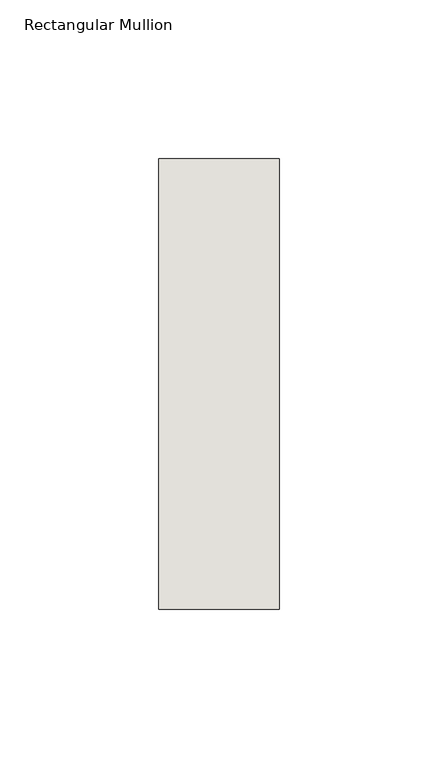
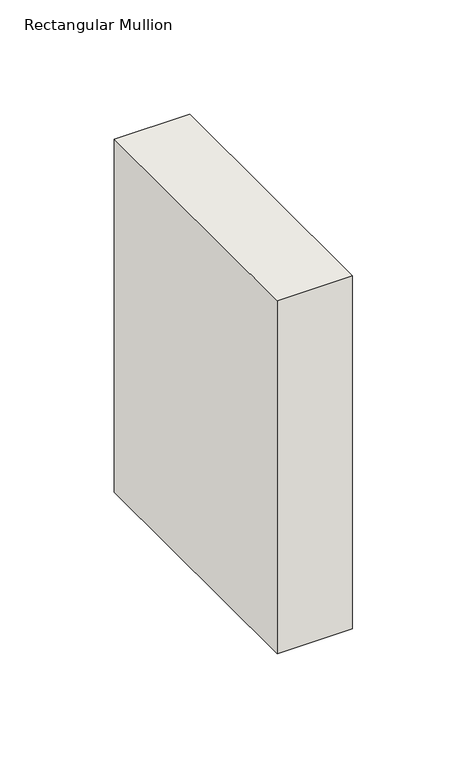
"""IFC4 building model written with IfcOpenShell, lengths in millimetres: wall geometry, Rectangular Mullion : NLRS_21_CWM_hsb-regel 38x142_gen_rsf."""

from ifc_helpers import new_model, si_unit, frame, origin, place, context, project, spatial, polyline, outline, extrude, source, transform, mapped, element, save


def rectangular_mullion_03fbd13c(model_context):
    return source(origin(), model_context, "Body", "SweptSolid", [
        extrude(outline(polyline([(0.0, -71.0), (-38.0, -71.0), (-38.0, 71.0), (0.0, 71.0), (0.0, -71.0)])), frame((0.0, 0.0, -188.0000003), z_axis=(0.0, 0.0, 1.0), x_axis=(1.0, 0.0, 0.0)), (0.0, 0.0, 1.0), 188.0000003),
    ])


if __name__ == "__main__":
    model = new_model("IFC4")
    model_context = context("Model", 3, world=origin())
    ifc_project = project(units=[si_unit("LENGTHUNIT", "METRE", prefix="MILLI")], contexts=[model_context])
    site = spatial("IfcSite", under=ifc_project)
    building = spatial("IfcBuilding", under=site)
    placement = place(None, origin())
    rectangular_mullion_shape = rectangular_mullion_03fbd13c(model_context)
    element("IfcWall", 1, ObjectType="Rectangular Mullion : NLRS_21_CWM_hsb-regel 38x142_gen_rsf", at=placement, inside=building, context=model_context, shape_type="MappedRepresentation", body=[
        mapped(rectangular_mullion_shape, transform((0.0, 0.0, 0.0), x_axis=(1.0, 0.0, 0.0), y_axis=(0.0, 1.0, 0.0), z_axis=(0.0, 0.0, 1.0))),
    ])
    save(model, "model.ifc")

# Revit data of these elements
# Type "Rectangular Mullion : NLRS_21_CWM_hsb-regel 38x142_gen_rsf"
#   Type IfcGUID = "07M7mRoiH1CR8m_RSKIwpF"
#   Assembly Code = "21.10"
#   IfcExportAs = "IfcWall"
#   built-in parameter 1007322 = 0.465879 (stored number, unit not read)
#   built-in parameter 1007321 = 0.062336 (stored number, unit not read)
#   built-in parameter 1007320 = 0.062336 (stored number, unit not read)
# Element 1 (IfcWall, "Rectangular Mullion : NLRS_21_CWM_hsb-regel 38x142_gen_rsf")
#   Materials on its faces: "NLRS_i2_hout naaldhout vuren_gen_rsf"
# Materials
#   "NLRS_i2_hout naaldhout vuren_gen_rsf": class "I - Hout", colour RGB 234 199 147, transparency 0, Keynote = "i2", Manufacturer = "Revit Standards Foundation", URL = "www.revitstandards.org", Description = "hout vuren", Cost = 0
